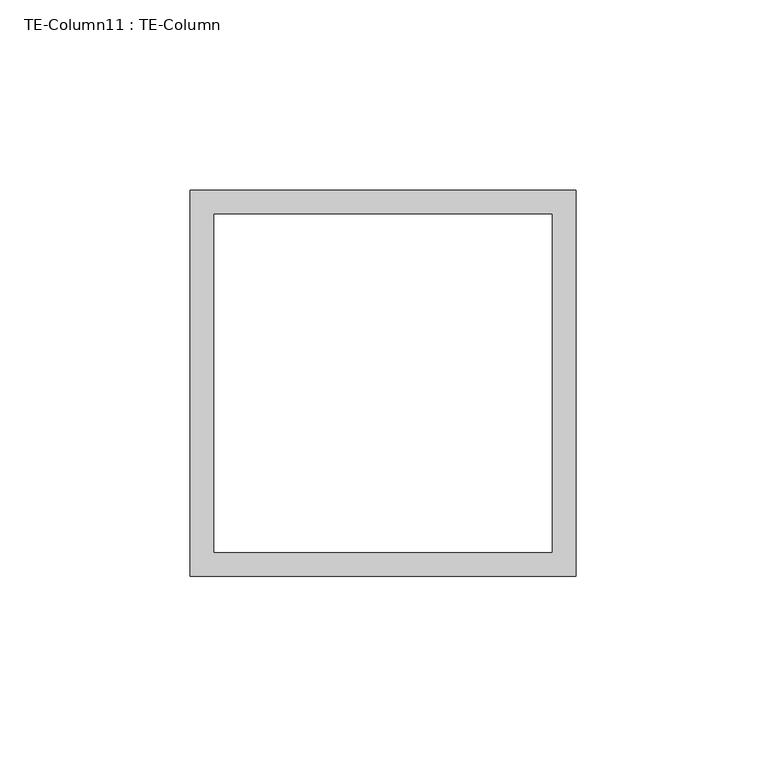
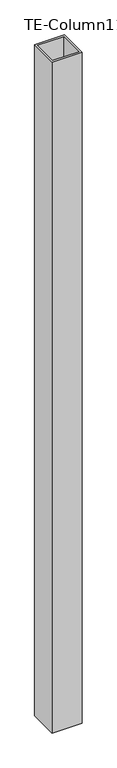
"""IFC4 building model written with IfcOpenShell, lengths in millimetres: proxy geometry, TE-Column11 : TE-Column."""

from ifc_helpers import new_model, si_unit, frame, origin, place, context, project, spatial, polyline, outline, extrude, source, transform, mapped, element, save


def te_column11_te_column_de7abfcb(model_context):
    return source(origin(), model_context, "Body", "SweptSolid", [
        extrude(outline(polyline([(588893.0684739, -531667.7913841), (588893.0684739, -531769.3913841), (588791.4684739, -531769.3913841), (588791.4684739, -531667.7913841), (588893.0684739, -531667.7913841)]), holes=[polyline([(588797.8184739, -531674.1413841), (588797.8184739, -531763.0413841), (588886.7184739, -531763.0413841), (588886.7184739, -531674.1413841), (588797.8184739, -531674.1413841)])]), frame((0.0, 0.0, 28.575), z_axis=(0.0, 0.0, 1.0), x_axis=(1.0, 0.0, 0.0)), (0.0, 0.0, 1.0), 2406.65),
    ])


if __name__ == "__main__":
    model = new_model("IFC4")
    model_context = context("Model", 3, world=origin())
    ifc_project = project(units=[si_unit("LENGTHUNIT", "METRE", prefix="MILLI")], contexts=[model_context])
    site = spatial("IfcSite", under=ifc_project)
    building = spatial("IfcBuilding", under=site)
    placement = place(None, origin())
    te_column11_te_column_shape = te_column11_te_column_de7abfcb(model_context)
    element("IfcBuildingElementProxy", 1, Name="TE-Column11 : TE-Column", ObjectType="TE-Column11 : TE-Column", at=placement, inside=building, context=model_context, shape_type="MappedRepresentation", body=[
        mapped(te_column11_te_column_shape, transform((0.0, 0.0, 0.0), x_axis=(1.0, 0.0, 0.0), y_axis=(0.0, 1.0, 0.0), z_axis=(0.0, 0.0, 1.0))),
    ])
    save(model, "model.ifc")

# Revit data of these elements
# Element 1 (IfcBuildingElementProxy, "TE-Column11 : TE-Column")
#   Materials on its faces: "4\"X4\" GALV. HSS TUBING"
# Materials
#   "4\"X4\" GALV. HSS TUBING": class "Generic", colour RGB 211 211 207, transparency 0, Cost = 0
